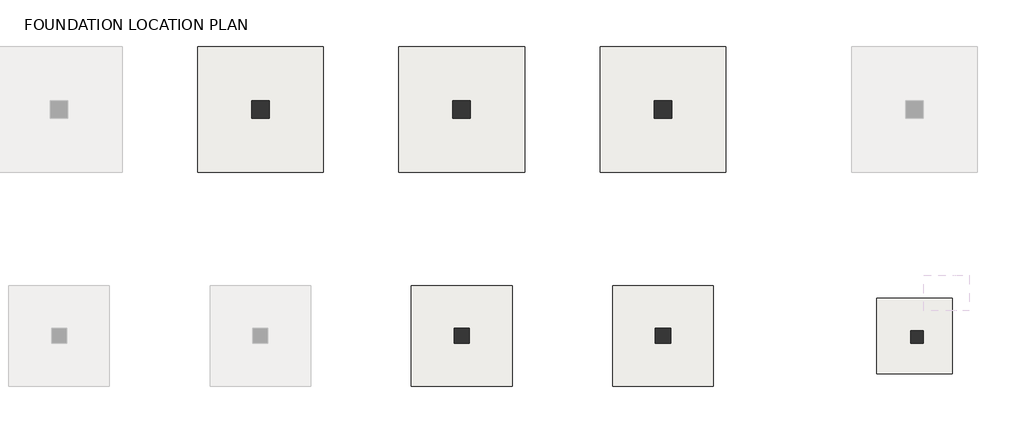
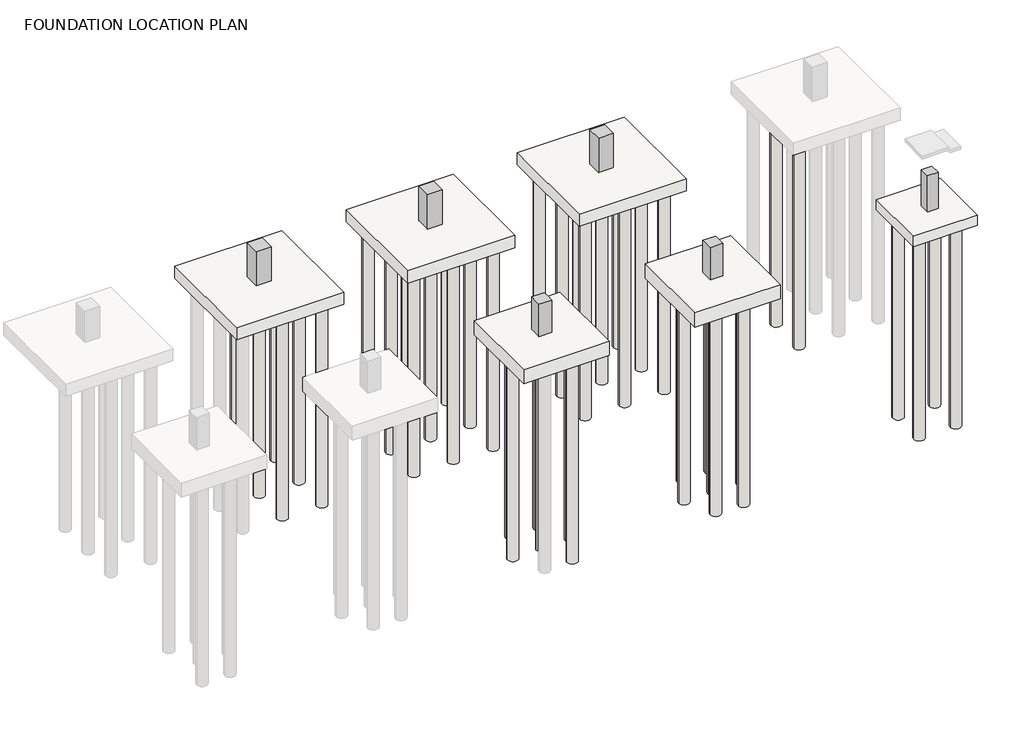
# One storey, part 2 of 3: 49 slabs, 6 columns.
"""IFC4 building model written with IfcOpenShell, lengths in millimetres."""

import ifcopenshell
import ifcopenshell.guid

model = None  # the IFC model being written
_history = None  # IfcOwnerHistory: only IFC2X3 demands one
_inside = {}  # id of a spatial element -> (the spatial element, [elements in it])
_under = {}  # id of a project, library or spatial element -> (it, [spatial elements below it])
_declared = {}  # id of a project -> (the project, [libraries it declares])
_typed = {}  # id of a type object -> (the type object, [elements of that type])
_made_of = {}  # id of a material, layer set ... -> (it, [elements and type objects made of it])


def new_model(schema):
    """Start an empty IFC model of exactly this schema.

    Asked for "IFC4X3", IfcOpenShell would pick the latest addendum, in which some entities
    have other attributes; the version numbers below select the first issue.
    IFC2X3 requires an IfcOwnerHistory on every rooted entity: one is made here for all.
    """
    global model, _history
    if schema == "IFC4X3":
        model = ifcopenshell.file(schema_version=(4, 3, 0, 0))
    else:
        model = ifcopenshell.file(schema=schema)
    _inside.clear()
    _under.clear()
    _declared.clear()
    _typed.clear()
    _made_of.clear()
    _history = None
    if model.schema == "IFC2X3":
        org = make("IfcOrganization", Name="unknown")
        user = make(
            "IfcPersonAndOrganization",
            ThePerson=make("IfcPerson", FamilyName="unknown"),
            TheOrganization=org,
        )
        app = make(
            "IfcApplication",
            ApplicationDeveloper=org,
            Version="unknown",
            ApplicationFullName="unknown",
            ApplicationIdentifier="unknown",
        )
        _history = make(
            "IfcOwnerHistory",
            OwningUser=user,
            OwningApplication=app,
            ChangeAction="ADDED",
            CreationDate=0,
        )
    return model


def make(cls, **values):
    """One entity of the class cls with the attributes given. An attribute that is None is left unset."""
    return model.create_entity(
        cls, **{name: value for name, value in values.items() if value is not None}
    )


def rooted(cls, **values):
    """An entity with a GlobalId (a new one), such as an element, a storey or a relation."""
    return make(cls, GlobalId=ifcopenshell.guid.new(), OwnerHistory=_history, **values)


def si_unit(unit_type, name, prefix=None):
    """IfcSIUnit, for example si_unit("LENGTHUNIT", "METRE", prefix="MILLI")."""
    return make("IfcSIUnit", UnitType=unit_type, Prefix=prefix, Name=name)


def assignment(units):
    """IfcUnitAssignment: the units of a project."""
    return None if units is None else make("IfcUnitAssignment", Units=units)


def point(xyz):
    """IfcCartesianPoint."""
    return None if xyz is None else make("IfcCartesianPoint", Coordinates=xyz)


def direction(xyz):
    """IfcDirection."""
    return None if xyz is None else make("IfcDirection", DirectionRatios=xyz)


def frame(location, z_axis=None, x_axis=None):
    """IfcAxis2Placement3D, a coordinate frame: its origin and axes. An axis left out is left unset."""
    return make(
        "IfcAxis2Placement3D",
        Location=point(location),
        Axis=direction(z_axis),
        RefDirection=direction(x_axis),
    )


def frame_2d(location, x_axis=None):
    """IfcAxis2Placement2D, a coordinate frame in the plane: its origin and x axis."""
    return make(
        "IfcAxis2Placement2D", Location=point(location), RefDirection=direction(x_axis)
    )


def origin():
    """The frame at (0, 0, 0) with its axes left unset."""
    return frame((0.0, 0.0, 0.0))


def place(relative_to, where):
    """IfcLocalPlacement: puts the frame where relative to a parent placement (None: the world)."""
    return make(
        "IfcLocalPlacement", PlacementRelTo=relative_to, RelativePlacement=where
    )


def context(
    kind, dimensions, precision=None, world=None, true_north=None, identifier=None
):
    """IfcGeometricRepresentationContext, for example the 3D "Model" context."""
    return make(
        "IfcGeometricRepresentationContext",
        ContextIdentifier=identifier,
        ContextType=kind,
        CoordinateSpaceDimension=dimensions,
        Precision=precision,
        WorldCoordinateSystem=world,
        TrueNorth=true_north,
    )


def project(units=None, contexts=None):
    """IfcProject with its units and contexts."""
    return rooted(
        "IfcProject",
        Name="project",
        RepresentationContexts=contexts,
        UnitsInContext=assignment(units),
    )


def spatial(cls, under=None, at=None, **own):
    """A site, building, storey or space (cls), placed at a placement, below another one or the project."""
    s = rooted(cls, ObjectPlacement=at, **own)
    if under is not None:
        _under.setdefault(under.id(), (under, []))[1].append(s)
    return s


def polyline(points):
    """IfcPolyline through the points."""
    return make("IfcPolyline", Points=[point(p) for p in points])


def circle_curve(where, radius):
    """IfcCircle in the frame where."""
    return make("IfcCircle", Position=where, Radius=radius)


def trimmed(basis, trim1, trim2, sense, master):
    """IfcTrimmedCurve: the piece of a basis curve between two trims."""
    return make(
        "IfcTrimmedCurve",
        BasisCurve=basis,
        Trim1=trim1,
        Trim2=trim2,
        SenseAgreement=sense,
        MasterRepresentation=master,
    )


def segment(curve, same_sense, transition):
    """IfcCompositeCurveSegment."""
    return make(
        "IfcCompositeCurveSegment",
        Transition=transition,
        SameSense=same_sense,
        ParentCurve=curve,
    )


def composite_curve(segments, self_intersect=None):
    """IfcCompositeCurve: segments joined end to end."""
    return make("IfcCompositeCurve", Segments=segments, SelfIntersect=self_intersect)


def outline(outer, holes=None, kind="AREA"):
    """IfcArbitraryClosedProfileDef: a profile drawn as a closed curve; with holes, ...WithVoids."""
    if holes is None:
        return make("IfcArbitraryClosedProfileDef", ProfileType=kind, OuterCurve=outer)
    return make(
        "IfcArbitraryProfileDefWithVoids",
        ProfileType=kind,
        OuterCurve=outer,
        InnerCurves=holes,
    )


def extrude(swept, where, along, depth):
    """IfcExtrudedAreaSolid: the profile swept, set in the frame where, extruded along a direction by depth."""
    return make(
        "IfcExtrudedAreaSolid",
        SweptArea=swept,
        Position=where,
        ExtrudedDirection=direction(along),
        Depth=depth,
    )


def faces_of(points, faces, orient=None, outer=None):
    """IfcFace entities. A face is a list of loops; a loop is a list of indices into points, from 0.

    orient and outer hold one flag for each loop. By default every Orientation is true, the
    first loop of a face is its IfcFaceOuterBound and the others are IfcFaceBound.
    """
    made = []
    for i, loops in enumerate(faces):
        bounds = []
        for j, loop in enumerate(loops):
            is_outer = j == 0 if outer is None else outer[i][j]
            bounds.append(
                make(
                    "IfcFaceOuterBound" if is_outer else "IfcFaceBound",
                    Bound=make("IfcPolyLoop", Polygon=[points[k] for k in loop]),
                    Orientation=True if orient is None else orient[i][j],
                )
            )
        made.append(make("IfcFace", Bounds=bounds))
    return made


def faceted_brep(points, faces, orient=None, outer=None, voids=None):
    """IfcFacetedBrep: a solid bounded by flat faces; with voids (closed shells), ...WithVoids."""
    shared = [point(p) for p in points]
    hull = make("IfcClosedShell", CfsFaces=faces_of(shared, faces, orient, outer))
    if voids is None:
        return make("IfcFacetedBrep", Outer=hull)
    return make(
        "IfcFacetedBrepWithVoids",
        Outer=hull,
        Voids=[
            make(cls, CfsFaces=faces_of(shared, fs, o, b)) for cls, fs, o, b in voids
        ],
    )


def shape(context_of_items, identifier, shape_type, items):
    """IfcShapeRepresentation: the items that make up one representation, for example the "Body"."""
    return make(
        "IfcShapeRepresentation",
        ContextOfItems=context_of_items,
        RepresentationIdentifier=identifier,
        RepresentationType=shape_type,
        Items=items,
    )


def made_of(thing, what):
    """Note that an element or type object is made of a material, layer set ...; save() writes the relation."""
    if what is not None:
        _made_of.setdefault(what.id(), (what, []))[1].append(thing)
    return thing


def element(
    cls,
    number,
    at=None,
    inside=None,
    cuts=None,
    type_object=None,
    material=None,
    context=None,
    identifier="Body",
    shape_type=None,
    held_by="IfcProductDefinitionShape",
    body=None,
    shapes=None,
    **own,
):
    """One element of the class cls, such as IfcWall. Its Tag is "e" and its number.

    at: its placement. inside: the storey or other place that contains it. cuts: it is an
    opening in that element (IfcRelVoidsElement). A single representation is given by context,
    identifier, shape_type and body (its items); several are given by shapes. held_by: the class
    of the entity that holds the representations. save() writes the other relations.
    """
    e = rooted(cls, Tag="e%d" % number, ObjectPlacement=at, **own)
    if body is not None:
        shapes = [shape(context, identifier, shape_type, body)]
    if shapes is not None:
        e.Representation = make(held_by, Representations=shapes)
    if inside is not None:
        _inside.setdefault(inside.id(), (inside, []))[1].append(e)
    if cuts is not None:
        rooted(
            "IfcRelVoidsElement", RelatingBuildingElement=cuts, RelatedOpeningElement=e
        )
    if type_object is not None:
        _typed.setdefault(type_object.id(), (type_object, []))[1].append(e)
    return made_of(e, material)


def aggregate(whole, parts):
    """IfcRelAggregates: a whole, such as a stair, and the parts it consists of."""
    return rooted("IfcRelAggregates", RelatingObject=whole, RelatedObjects=parts)


def save(model, path):
    """Write the relations noted so far, then the file.

    IfcRelAggregates (storeys below a building ...), IfcRelContainedInSpatialStructure (elements
    in a storey), IfcRelDefinesByType, IfcRelAssociatesMaterial and IfcRelDeclares: one each for
    every whole, place, type object, material and project.
    """
    for whole, parts in _under.values():
        aggregate(whole, parts)
    for where, things in _inside.values():
        rooted(
            "IfcRelContainedInSpatialStructure",
            RelatedElements=things,
            RelatingStructure=where,
        )
    for kind, things in _typed.values():
        rooted("IfcRelDefinesByType", RelatedObjects=things, RelatingType=kind)
    for what, things in _made_of.values():
        rooted("IfcRelAssociatesMaterial", RelatedObjects=things, RelatingMaterial=what)
    for by, libraries in _declared.values():
        rooted("IfcRelDeclares", RelatingContext=by, RelatedDefinitions=libraries)
    model.write(path)


model = new_model("IFC4")

# Units and contexts
model_context = context("Model", 3, world=origin())
ifc_project = project(units=[si_unit("LENGTHUNIT", "METRE", prefix="MILLI")], contexts=[model_context])

# Site, building, storey
site = spatial("IfcSite", under=ifc_project)
building = spatial("IfcBuilding", under=site)
storey = spatial("IfcBuildingStorey", under=building, Name="FOUNDATION LOCATION PLAN", Elevation=-1699.994759)

# Columns
placement = place(None, origin())
element("IfcColumn", 1, ObjectType="Concrete-Rectangular-Column_R1 : CLS111_RC COLUMN_UG_C1", at=placement, inside=storey, context=model_context, shape_type="Brep", body=[
    faceted_brep([(41850.0, 21199.5208589, -1199.994759), (42350.0, 21199.5208589, -1199.994759), (42350.0, 20699.5208589, -1199.994759), (41850.0, 20699.5208589, -1199.994759), (41850.0, 21199.5208589, 450.005241), (41850.0, 21199.5208589, 600.005241), (42000.0, 21199.5208589, 600.005241), (42350.0, 21199.5208589, 600.005241), (41850.0, 20699.5208589, 600.005241), (41850.0, 20999.5208589, 600.005241), (42350.0, 20699.5208589, 600.005241)], [[[0, 1, 2, 3]], [[1, 0, 4, 5, 6, 7]], [[0, 3, 8, 9, 5, 4]], [[3, 2, 10, 8]], [[2, 1, 7, 10]], [[8, 10, 7, 6, 5, 9]]]),
])
element("IfcColumn", 2, ObjectType="Concrete-Rectangular-Column_R1 : CLS111_RC COLUMN_UG_C3", at=placement, inside=storey, context=model_context, shape_type="Brep", body=[
    faceted_brep([(15650.0, 30349.5208589, -1099.994759), (16350.0, 30349.5208589, -1099.994759), (16350.0, 29649.5208589, -1099.994759), (15650.0, 29649.5208589, -1099.994759), (15650.0, 30349.5208589, 450.005241), (15650.0, 30349.5208589, 600.005241), (16350.0, 30349.5208589, 600.005241), (16350.0, 30349.5208589, 450.005241), (16350.0, 29649.5208589, 600.005241), (16350.0, 29649.5208589, 450.005241), (15650.0, 29649.5208589, 600.005241), (15650.0, 29649.5208589, 450.005241)], [[[0, 1, 2, 3]], [[1, 0, 4, 5, 6, 7]], [[2, 1, 7, 6, 8, 9]], [[3, 2, 9, 8, 10, 11]], [[0, 3, 11, 10, 5, 4]], [[6, 5, 10, 8]]]),
])
element("IfcColumn", 3, ObjectType="Concrete-Rectangular-Column_R1 : CLS111_RC COLUMN_UG_C3", at=placement, inside=storey, context=model_context, shape_type="Brep", body=[
    faceted_brep([(23650.0, 30349.5208589, -1099.994759), (24350.0, 30349.5208589, -1099.994759), (24350.0, 29649.5208589, -1099.994759), (23650.0, 29649.5208589, -1099.994759), (23650.0, 30349.5208589, 450.005241), (23650.0, 30349.5208589, 600.005241), (24350.0, 30349.5208589, 600.005241), (24350.0, 30349.5208589, 450.005241), (24350.0, 29649.5208589, 600.005241), (24350.0, 29649.5208589, 450.005241), (23650.0, 29649.5208589, 600.005241), (23650.0, 29649.5208589, 450.005241)], [[[0, 1, 2, 3]], [[1, 0, 4, 5, 6, 7]], [[2, 1, 7, 6, 8, 9]], [[3, 2, 9, 8, 10, 11]], [[0, 3, 11, 10, 5, 4]], [[6, 5, 10, 8]]]),
])
element("IfcColumn", 4, ObjectType="Concrete-Rectangular-Column_R1 : CLS111_RC COLUMN_UG_C3", at=placement, inside=storey, context=model_context, shape_type="Brep", body=[
    faceted_brep([(31650.0, 30349.5208589, -1099.994759), (32350.0, 30349.5208589, -1099.994759), (32350.0, 29649.5208589, -1099.994759), (31650.0, 29649.5208589, -1099.994759), (31650.0, 30349.5208589, 450.005241), (31650.0, 30349.5208589, 600.005241), (32350.0, 30349.5208589, 600.005241), (32350.0, 30349.5208589, 450.005241), (32350.0, 29649.5208589, 600.005241), (32350.0, 29649.5208589, 450.005241), (31650.0, 29649.5208589, 600.005241), (31650.0, 29649.5208589, 450.005241)], [[[0, 1, 2, 3]], [[1, 0, 4, 5, 6, 7]], [[2, 1, 7, 6, 8, 9]], [[3, 2, 9, 8, 10, 11]], [[0, 3, 11, 10, 5, 4]], [[6, 5, 10, 8]]]),
])
element("IfcColumn", 5, ObjectType="Concrete-Rectangular-Column_R1 : CLS111_RC COLUMN_UG_C2", at=placement, inside=storey, context=model_context, shape_type="Brep", body=[
    faceted_brep([(23700.0, 21299.5208589, -999.994759), (24300.0, 21299.5208589, -999.994759), (24300.0, 20699.5208589, -999.994759), (23700.0, 20699.5208589, -999.994759), (23700.0, 21299.5208589, 450.005241), (23700.0, 21299.5208589, 600.005241), (24300.0, 21299.5208589, 600.005241), (24300.0, 21299.5208589, 450.005241), (24300.0, 20999.5208589, 600.005241), (24300.0, 20699.5208589, 600.005241), (23700.0, 20699.5208589, 600.005241), (23700.0, 20999.5208589, 600.005241)], [[[0, 1, 2, 3]], [[1, 0, 4, 5, 6, 7]], [[2, 1, 7, 6, 8, 9]], [[3, 2, 9, 10]], [[0, 3, 10, 11, 5, 4]], [[6, 5, 11, 10, 9, 8]]]),
])
element("IfcColumn", 6, ObjectType="Concrete-Rectangular-Column_R1 : CLS111_RC COLUMN_UG_C2", at=placement, inside=storey, context=model_context, shape_type="Brep", body=[
    faceted_brep([(31700.0, 21299.5208589, -999.994759), (32300.0, 21299.5208589, -999.994759), (32300.0, 20699.5208589, -999.994759), (31700.0, 20699.5208589, -999.994759), (31700.0, 21299.5208589, 450.005241), (31700.0, 21299.5208589, 600.005241), (32300.0, 21299.5208589, 600.005241), (32300.0, 21299.5208589, 450.005241), (32300.0, 20999.5208589, 600.005241), (32300.0, 20699.5208589, 600.005241), (31700.0, 20699.5208589, 600.005241), (31700.0, 20999.5208589, 600.005241)], [[[0, 1, 2, 3]], [[1, 0, 4, 5, 6, 7]], [[2, 1, 7, 6, 8, 9]], [[3, 2, 9, 10]], [[0, 3, 10, 11, 5, 4]], [[6, 5, 11, 10, 9, 8]]]),
])

# Slabs
element("IfcSlab", 7, ObjectType="Footing-Rectangular_R1 : FTS301_Footing-Rectangular_3000x3000x500_F1", at=placement, inside=storey, context=model_context, shape_type="SweptSolid", body=[
    extrude(outline(polyline([(43500.0, 22499.5208589), (43500.0, 19499.5208589), (40500.0, 19499.5208589), (40500.0, 22499.5208589), (43500.0, 22499.5208589)])), frame((0.0, 0.0, -1699.994759), z_axis=(0.0, 0.0, 1.0), x_axis=(1.0, 0.0, 0.0)), (0.0, 0.0, 1.0), 500.0),
])
element("IfcSlab", 8, ObjectType="Footing-Rectangular_R1 : FTS301_Footing-Rectangular_4000x4000x700_F2", at=placement, inside=storey, context=model_context, shape_type="SweptSolid", body=[
    extrude(outline(polyline([(26000.0, 22999.5208589), (26000.0, 18999.5208589), (22000.0, 18999.5208589), (22000.0, 22999.5208589), (26000.0, 22999.5208589)])), frame((0.0, 0.0, -1699.994759), z_axis=(0.0, 0.0, 1.0), x_axis=(1.0, 0.0, 0.0)), (0.0, 0.0, 1.0), 700.0),
])
element("IfcSlab", 9, ObjectType="Footing-Rectangular_R1 : FTS301_Footing-Rectangular_4000x4000x700_F2", at=placement, inside=storey, context=model_context, shape_type="SweptSolid", body=[
    extrude(outline(polyline([(34000.0, 22999.5208589), (34000.0, 18999.5208589), (30000.0, 18999.5208589), (30000.0, 22999.5208589), (34000.0, 22999.5208589)])), frame((0.0, 0.0, -1699.994759), z_axis=(0.0, 0.0, 1.0), x_axis=(1.0, 0.0, 0.0)), (0.0, 0.0, 1.0), 700.0),
])
element("IfcSlab", 10, ObjectType="Footing-Rectangular_R1 : FTS301_Footing-Rectangular_5000x5000x600_F3", at=placement, inside=storey, context=model_context, shape_type="SweptSolid", body=[
    extrude(outline(polyline([(18500.0, 32499.5208589), (18500.0, 27499.5208589), (13500.0, 27499.5208589), (13500.0, 32499.5208589), (18500.0, 32499.5208589)])), frame((0.0, 0.0, -1699.994759), z_axis=(0.0, 0.0, 1.0), x_axis=(1.0, 0.0, 0.0)), (0.0, 0.0, 1.0), 600.0),
])
element("IfcSlab", 11, ObjectType="Footing-Rectangular_R1 : FTS301_Footing-Rectangular_5000x5000x600_F3", at=placement, inside=storey, context=model_context, shape_type="SweptSolid", body=[
    extrude(outline(polyline([(26500.0, 32499.5208589), (26500.0, 27499.5208589), (21500.0, 27499.5208589), (21500.0, 32499.5208589), (26500.0, 32499.5208589)])), frame((0.0, 0.0, -1699.994759), z_axis=(0.0, 0.0, 1.0), x_axis=(1.0, 0.0, 0.0)), (0.0, 0.0, 1.0), 600.0),
])
element("IfcSlab", 12, ObjectType="Footing-Rectangular_R1 : FTS301_Footing-Rectangular_5000x5000x600_F3", at=placement, inside=storey, context=model_context, shape_type="SweptSolid", body=[
    extrude(outline(polyline([(34500.0, 32499.5208589), (34500.0, 27499.5208589), (29500.0, 27499.5208589), (29500.0, 32499.5208589), (34500.0, 32499.5208589)])), frame((0.0, 0.0, -1699.994759), z_axis=(0.0, 0.0, 1.0), x_axis=(1.0, 0.0, 0.0)), (0.0, 0.0, 1.0), 600.0),
])
element("IfcSlab", 13, ObjectType="HEC_PILE : FTPS102_D500", at=placement, inside=storey, context=model_context, shape_type="SweptSolid", body=[
    extrude(outline(composite_curve([segment(trimmed(circle_curve(frame_2d((41150.0, 21849.5208589)), 250.0), [point((41400.0, 21849.5208589))], [point((40900.0, 21849.5208589))], False, "CARTESIAN"), True, "CONTINUOUS"), segment(trimmed(circle_curve(frame_2d((41150.0, 21849.5208589)), 250.0), [point((40900.0, 21849.5208589))], [point((41400.0, 21849.5208589))], False, "CARTESIAN"), True, "CONTINUOUS")], self_intersect=False)), frame((0.0, 0.0, -11749.994759), z_axis=(0.0, 0.0, 1.0), x_axis=(1.0, 0.0, 0.0)), (0.0, 0.0, 1.0), 10150.0),
])
element("IfcSlab", 14, ObjectType="HEC_PILE : FTPS102_D500", at=placement, inside=storey, context=model_context, shape_type="SweptSolid", body=[
    extrude(outline(composite_curve([segment(trimmed(circle_curve(frame_2d((42850.0, 21849.5208589)), 250.0), [point((42600.0, 21849.5208589))], [point((43100.0, 21849.5208589))], False, "CARTESIAN"), True, "CONTINUOUS"), segment(trimmed(circle_curve(frame_2d((42850.0, 21849.5208589)), 250.0), [point((43100.0, 21849.5208589))], [point((42600.0, 21849.5208589))], False, "CARTESIAN"), True, "CONTINUOUS")], self_intersect=False)), frame((0.0, 0.0, -11749.994759), z_axis=(0.0, 0.0, 1.0), x_axis=(1.0, 0.0, 0.0)), (0.0, 0.0, 1.0), 10150.0),
])
element("IfcSlab", 15, ObjectType="HEC_PILE : FTPS102_D500", at=placement, inside=storey, context=model_context, shape_type="SweptSolid", body=[
    extrude(outline(composite_curve([segment(trimmed(circle_curve(frame_2d((41150.0, 20149.5208589)), 250.0), [point((41400.0, 20149.5208589))], [point((40900.0, 20149.5208589))], False, "CARTESIAN"), True, "CONTINUOUS"), segment(trimmed(circle_curve(frame_2d((41150.0, 20149.5208589)), 250.0), [point((40900.0, 20149.5208589))], [point((41400.0, 20149.5208589))], False, "CARTESIAN"), True, "CONTINUOUS")], self_intersect=False)), frame((0.0, 0.0, -11749.994759), z_axis=(0.0, 0.0, 1.0), x_axis=(1.0, 0.0, 0.0)), (0.0, 0.0, 1.0), 10150.0),
])
element("IfcSlab", 16, ObjectType="HEC_PILE : FTPS102_D500", at=placement, inside=storey, context=model_context, shape_type="SweptSolid", body=[
    extrude(outline(composite_curve([segment(trimmed(circle_curve(frame_2d((42850.0, 20149.5208589)), 250.0), [point((42600.0, 20149.5208589))], [point((43100.0, 20149.5208589))], False, "CARTESIAN"), True, "CONTINUOUS"), segment(trimmed(circle_curve(frame_2d((42850.0, 20149.5208589)), 250.0), [point((43100.0, 20149.5208589))], [point((42600.0, 20149.5208589))], False, "CARTESIAN"), True, "CONTINUOUS")], self_intersect=False)), frame((0.0, 0.0, -11749.994759), z_axis=(0.0, 0.0, 1.0), x_axis=(1.0, 0.0, 0.0)), (0.0, 0.0, 1.0), 10150.0),
])
element("IfcSlab", 17, ObjectType="HEC_PILE : FTPS102_D500", at=placement, inside=storey, context=model_context, shape_type="SweptSolid", body=[
    extrude(outline(composite_curve([segment(trimmed(circle_curve(frame_2d((24650.0, 19649.5208589)), 250.0), [point((24400.0, 19649.5208589))], [point((24900.0, 19649.5208589))], False, "CARTESIAN"), True, "CONTINUOUS"), segment(trimmed(circle_curve(frame_2d((24650.0, 19649.5208589)), 250.0), [point((24900.0, 19649.5208589))], [point((24400.0, 19649.5208589))], False, "CARTESIAN"), True, "CONTINUOUS")], self_intersect=False)), frame((0.0, 0.0, -11749.994759), z_axis=(0.0, 0.0, 1.0), x_axis=(1.0, 0.0, 0.0)), (0.0, 0.0, 1.0), 10150.0),
])
element("IfcSlab", 18, ObjectType="HEC_PILE : FTPS102_D500", at=placement, inside=storey, context=model_context, shape_type="SweptSolid", body=[
    extrude(outline(composite_curve([segment(trimmed(circle_curve(frame_2d((22650.0, 20999.5208589)), 250.0), [point((22900.0, 20999.5208589))], [point((22400.0, 20999.5208589))], False, "CARTESIAN"), True, "CONTINUOUS"), segment(trimmed(circle_curve(frame_2d((22650.0, 20999.5208589)), 250.0), [point((22400.0, 20999.5208589))], [point((22900.0, 20999.5208589))], False, "CARTESIAN"), True, "CONTINUOUS")], self_intersect=False)), frame((0.0, 0.0, -11749.994759), z_axis=(0.0, 0.0, 1.0), x_axis=(1.0, 0.0, 0.0)), (0.0, 0.0, 1.0), 10150.0),
])
element("IfcSlab", 19, ObjectType="HEC_PILE : FTPS102_D500", at=placement, inside=storey, context=model_context, shape_type="SweptSolid", body=[
    extrude(outline(composite_curve([segment(trimmed(circle_curve(frame_2d((24000.0, 20999.5208589)), 250.0), [point((24250.0, 20999.5208589))], [point((23750.0, 20999.5208589))], False, "CARTESIAN"), True, "CONTINUOUS"), segment(trimmed(circle_curve(frame_2d((24000.0, 20999.5208589)), 250.0), [point((23750.0, 20999.5208589))], [point((24250.0, 20999.5208589))], False, "CARTESIAN"), True, "CONTINUOUS")], self_intersect=False)), frame((0.0, 0.0, -11749.994759), z_axis=(0.0, 0.0, 1.0), x_axis=(1.0, 0.0, 0.0)), (0.0, 0.0, 1.0), 10150.0),
])
element("IfcSlab", 20, ObjectType="HEC_PILE : FTPS102_D500", at=placement, inside=storey, context=model_context, shape_type="SweptSolid", body=[
    extrude(outline(composite_curve([segment(trimmed(circle_curve(frame_2d((25350.0, 20999.5208589)), 250.0), [point((25100.0, 20999.5208589))], [point((25600.0, 20999.5208589))], False, "CARTESIAN"), True, "CONTINUOUS"), segment(trimmed(circle_curve(frame_2d((25350.0, 20999.5208589)), 250.0), [point((25600.0, 20999.5208589))], [point((25100.0, 20999.5208589))], False, "CARTESIAN"), True, "CONTINUOUS")], self_intersect=False)), frame((0.0, 0.0, -11749.994759), z_axis=(0.0, 0.0, 1.0), x_axis=(1.0, 0.0, 0.0)), (0.0, 0.0, 1.0), 10150.0),
])
element("IfcSlab", 21, ObjectType="HEC_PILE : FTPS102_D500", at=placement, inside=storey, context=model_context, shape_type="SweptSolid", body=[
    extrude(outline(composite_curve([segment(trimmed(circle_curve(frame_2d((23350.0, 22349.5208589)), 250.0), [point((23600.0, 22349.5208589))], [point((23100.0, 22349.5208589))], False, "CARTESIAN"), True, "CONTINUOUS"), segment(trimmed(circle_curve(frame_2d((23350.0, 22349.5208589)), 250.0), [point((23100.0, 22349.5208589))], [point((23600.0, 22349.5208589))], False, "CARTESIAN"), True, "CONTINUOUS")], self_intersect=False)), frame((0.0, 0.0, -11749.994759), z_axis=(0.0, 0.0, 1.0), x_axis=(1.0, 0.0, 0.0)), (0.0, 0.0, 1.0), 10150.0),
])
element("IfcSlab", 22, ObjectType="HEC_PILE : FTPS102_D500", at=placement, inside=storey, context=model_context, shape_type="SweptSolid", body=[
    extrude(outline(composite_curve([segment(trimmed(circle_curve(frame_2d((24650.0, 22349.5208589)), 250.0), [point((24400.0, 22349.5208589))], [point((24900.0, 22349.5208589))], False, "CARTESIAN"), True, "CONTINUOUS"), segment(trimmed(circle_curve(frame_2d((24650.0, 22349.5208589)), 250.0), [point((24900.0, 22349.5208589))], [point((24400.0, 22349.5208589))], False, "CARTESIAN"), True, "CONTINUOUS")], self_intersect=False)), frame((0.0, 0.0, -11749.994759), z_axis=(0.0, 0.0, 1.0), x_axis=(1.0, 0.0, 0.0)), (0.0, 0.0, 1.0), 10150.0),
])
element("IfcSlab", 23, ObjectType="HEC_PILE : FTPS102_D500", at=placement, inside=storey, context=model_context, shape_type="SweptSolid", body=[
    extrude(outline(composite_curve([segment(trimmed(circle_curve(frame_2d((31350.0, 19649.5208589)), 250.0), [point((31600.0, 19649.5208589))], [point((31100.0, 19649.5208589))], False, "CARTESIAN"), True, "CONTINUOUS"), segment(trimmed(circle_curve(frame_2d((31350.0, 19649.5208589)), 250.0), [point((31100.0, 19649.5208589))], [point((31600.0, 19649.5208589))], False, "CARTESIAN"), True, "CONTINUOUS")], self_intersect=False)), frame((0.0, 0.0, -11749.994759), z_axis=(0.0, 0.0, 1.0), x_axis=(1.0, 0.0, 0.0)), (0.0, 0.0, 1.0), 10150.0),
])
element("IfcSlab", 24, ObjectType="HEC_PILE : FTPS102_D500", at=placement, inside=storey, context=model_context, shape_type="SweptSolid", body=[
    extrude(outline(composite_curve([segment(trimmed(circle_curve(frame_2d((32650.0, 19649.5208589)), 250.0), [point((32400.0, 19649.5208589))], [point((32900.0, 19649.5208589))], False, "CARTESIAN"), True, "CONTINUOUS"), segment(trimmed(circle_curve(frame_2d((32650.0, 19649.5208589)), 250.0), [point((32900.0, 19649.5208589))], [point((32400.0, 19649.5208589))], False, "CARTESIAN"), True, "CONTINUOUS")], self_intersect=False)), frame((0.0, 0.0, -11749.994759), z_axis=(0.0, 0.0, 1.0), x_axis=(1.0, 0.0, 0.0)), (0.0, 0.0, 1.0), 10150.0),
])
element("IfcSlab", 25, ObjectType="HEC_PILE : FTPS102_D500", at=placement, inside=storey, context=model_context, shape_type="SweptSolid", body=[
    extrude(outline(composite_curve([segment(trimmed(circle_curve(frame_2d((30650.0, 20999.5208589)), 250.0), [point((30900.0, 20999.5208589))], [point((30400.0, 20999.5208589))], False, "CARTESIAN"), True, "CONTINUOUS"), segment(trimmed(circle_curve(frame_2d((30650.0, 20999.5208589)), 250.0), [point((30400.0, 20999.5208589))], [point((30900.0, 20999.5208589))], False, "CARTESIAN"), True, "CONTINUOUS")], self_intersect=False)), frame((0.0, 0.0, -11749.994759), z_axis=(0.0, 0.0, 1.0), x_axis=(1.0, 0.0, 0.0)), (0.0, 0.0, 1.0), 10150.0),
])
element("IfcSlab", 26, ObjectType="HEC_PILE : FTPS102_D500", at=placement, inside=storey, context=model_context, shape_type="SweptSolid", body=[
    extrude(outline(composite_curve([segment(trimmed(circle_curve(frame_2d((32000.0, 20999.5208589)), 250.0), [point((32250.0, 20999.5208589))], [point((31750.0, 20999.5208589))], False, "CARTESIAN"), True, "CONTINUOUS"), segment(trimmed(circle_curve(frame_2d((32000.0, 20999.5208589)), 250.0), [point((31750.0, 20999.5208589))], [point((32250.0, 20999.5208589))], False, "CARTESIAN"), True, "CONTINUOUS")], self_intersect=False)), frame((0.0, 0.0, -11749.994759), z_axis=(0.0, 0.0, 1.0), x_axis=(1.0, 0.0, 0.0)), (0.0, 0.0, 1.0), 10150.0),
])
element("IfcSlab", 27, ObjectType="HEC_PILE : FTPS102_D500", at=placement, inside=storey, context=model_context, shape_type="SweptSolid", body=[
    extrude(outline(composite_curve([segment(trimmed(circle_curve(frame_2d((33350.0, 20999.5208589)), 250.0), [point((33100.0, 20999.5208589))], [point((33600.0, 20999.5208589))], False, "CARTESIAN"), True, "CONTINUOUS"), segment(trimmed(circle_curve(frame_2d((33350.0, 20999.5208589)), 250.0), [point((33600.0, 20999.5208589))], [point((33100.0, 20999.5208589))], False, "CARTESIAN"), True, "CONTINUOUS")], self_intersect=False)), frame((0.0, 0.0, -11749.994759), z_axis=(0.0, 0.0, 1.0), x_axis=(1.0, 0.0, 0.0)), (0.0, 0.0, 1.0), 10150.0),
])
element("IfcSlab", 28, ObjectType="HEC_PILE : FTPS102_D500", at=placement, inside=storey, context=model_context, shape_type="SweptSolid", body=[
    extrude(outline(composite_curve([segment(trimmed(circle_curve(frame_2d((31350.0, 22349.5208589)), 250.0), [point((31600.0, 22349.5208589))], [point((31100.0, 22349.5208589))], False, "CARTESIAN"), True, "CONTINUOUS"), segment(trimmed(circle_curve(frame_2d((31350.0, 22349.5208589)), 250.0), [point((31100.0, 22349.5208589))], [point((31600.0, 22349.5208589))], False, "CARTESIAN"), True, "CONTINUOUS")], self_intersect=False)), frame((0.0, 0.0, -11749.994759), z_axis=(0.0, 0.0, 1.0), x_axis=(1.0, 0.0, 0.0)), (0.0, 0.0, 1.0), 10150.0),
])
element("IfcSlab", 29, ObjectType="HEC_PILE : FTPS102_D500", at=placement, inside=storey, context=model_context, shape_type="SweptSolid", body=[
    extrude(outline(composite_curve([segment(trimmed(circle_curve(frame_2d((32650.0, 22349.5208589)), 250.0), [point((32400.0, 22349.5208589))], [point((32900.0, 22349.5208589))], False, "CARTESIAN"), True, "CONTINUOUS"), segment(trimmed(circle_curve(frame_2d((32650.0, 22349.5208589)), 250.0), [point((32900.0, 22349.5208589))], [point((32400.0, 22349.5208589))], False, "CARTESIAN"), True, "CONTINUOUS")], self_intersect=False)), frame((0.0, 0.0, -11749.994759), z_axis=(0.0, 0.0, 1.0), x_axis=(1.0, 0.0, 0.0)), (0.0, 0.0, 1.0), 10150.0),
])
element("IfcSlab", 30, ObjectType="HEC_PILE : FTPS102_D500", at=placement, inside=storey, context=model_context, shape_type="SweptSolid", body=[
    extrude(outline(composite_curve([segment(trimmed(circle_curve(frame_2d((17850.0, 29999.5208589)), 250.0), [point((17600.0, 29999.5208589))], [point((18100.0, 29999.5208589))], False, "CARTESIAN"), True, "CONTINUOUS"), segment(trimmed(circle_curve(frame_2d((17850.0, 29999.5208589)), 250.0), [point((18100.0, 29999.5208589))], [point((17600.0, 29999.5208589))], False, "CARTESIAN"), True, "CONTINUOUS")], self_intersect=False)), frame((0.0, 0.0, -11749.994759), z_axis=(0.0, 0.0, 1.0), x_axis=(1.0, 0.0, 0.0)), (0.0, 0.0, 1.0), 10150.0),
])
element("IfcSlab", 31, ObjectType="HEC_PILE : FTPS102_D500", at=placement, inside=storey, context=model_context, shape_type="SweptSolid", body=[
    extrude(outline(composite_curve([segment(trimmed(circle_curve(frame_2d((16000.0, 29999.5208589)), 250.0), [point((15750.0, 29999.5208589))], [point((16250.0, 29999.5208589))], False, "CARTESIAN"), True, "CONTINUOUS"), segment(trimmed(circle_curve(frame_2d((16000.0, 29999.5208589)), 250.0), [point((16250.0, 29999.5208589))], [point((15750.0, 29999.5208589))], False, "CARTESIAN"), True, "CONTINUOUS")], self_intersect=False)), frame((0.0, 0.0, -11749.994759), z_axis=(0.0, 0.0, 1.0), x_axis=(1.0, 0.0, 0.0)), (0.0, 0.0, 1.0), 10150.0),
])
element("IfcSlab", 32, ObjectType="HEC_PILE : FTPS102_D500", at=placement, inside=storey, context=model_context, shape_type="SweptSolid", body=[
    extrude(outline(composite_curve([segment(trimmed(circle_curve(frame_2d((17850.0, 31849.5208589)), 250.0), [point((17600.0, 31849.5208589))], [point((18100.0, 31849.5208589))], False, "CARTESIAN"), True, "CONTINUOUS"), segment(trimmed(circle_curve(frame_2d((17850.0, 31849.5208589)), 250.0), [point((18100.0, 31849.5208589))], [point((17600.0, 31849.5208589))], False, "CARTESIAN"), True, "CONTINUOUS")], self_intersect=False)), frame((0.0, 0.0, -11749.994759), z_axis=(0.0, 0.0, 1.0), x_axis=(1.0, 0.0, 0.0)), (0.0, 0.0, 1.0), 10150.0),
])
element("IfcSlab", 33, ObjectType="HEC_PILE : FTPS102_D500", at=placement, inside=storey, context=model_context, shape_type="SweptSolid", body=[
    extrude(outline(composite_curve([segment(trimmed(circle_curve(frame_2d((16000.0, 31849.5208589)), 250.0), [point((15750.0, 31849.5208589))], [point((16250.0, 31849.5208589))], False, "CARTESIAN"), True, "CONTINUOUS"), segment(trimmed(circle_curve(frame_2d((16000.0, 31849.5208589)), 250.0), [point((16250.0, 31849.5208589))], [point((15750.0, 31849.5208589))], False, "CARTESIAN"), True, "CONTINUOUS")], self_intersect=False)), frame((0.0, 0.0, -11749.994759), z_axis=(0.0, 0.0, 1.0), x_axis=(1.0, 0.0, 0.0)), (0.0, 0.0, 1.0), 10150.0),
])
element("IfcSlab", 34, ObjectType="HEC_PILE : FTPS102_D500", at=placement, inside=storey, context=model_context, shape_type="SweptSolid", body=[
    extrude(outline(composite_curve([segment(trimmed(circle_curve(frame_2d((17850.0, 28149.5208589)), 250.0), [point((17600.0, 28149.5208589))], [point((18100.0, 28149.5208589))], False, "CARTESIAN"), True, "CONTINUOUS"), segment(trimmed(circle_curve(frame_2d((17850.0, 28149.5208589)), 250.0), [point((18100.0, 28149.5208589))], [point((17600.0, 28149.5208589))], False, "CARTESIAN"), True, "CONTINUOUS")], self_intersect=False)), frame((0.0, 0.0, -11749.994759), z_axis=(0.0, 0.0, 1.0), x_axis=(1.0, 0.0, 0.0)), (0.0, 0.0, 1.0), 10150.0),
])
element("IfcSlab", 35, ObjectType="HEC_PILE : FTPS102_D500", at=placement, inside=storey, context=model_context, shape_type="SweptSolid", body=[
    extrude(outline(composite_curve([segment(trimmed(circle_curve(frame_2d((16000.0, 28149.5208589)), 250.0), [point((15750.0, 28149.5208589))], [point((16250.0, 28149.5208589))], False, "CARTESIAN"), True, "CONTINUOUS"), segment(trimmed(circle_curve(frame_2d((16000.0, 28149.5208589)), 250.0), [point((16250.0, 28149.5208589))], [point((15750.0, 28149.5208589))], False, "CARTESIAN"), True, "CONTINUOUS")], self_intersect=False)), frame((0.0, 0.0, -11749.994759), z_axis=(0.0, 0.0, 1.0), x_axis=(1.0, 0.0, 0.0)), (0.0, 0.0, 1.0), 10150.0),
])
element("IfcSlab", 36, ObjectType="HEC_PILE : FTPS102_D500", at=placement, inside=storey, context=model_context, shape_type="SweptSolid", body=[
    extrude(outline(composite_curve([segment(trimmed(circle_curve(frame_2d((22150.0, 29999.5208589)), 250.0), [point((22400.0, 29999.5208589))], [point((21900.0, 29999.5208589))], False, "CARTESIAN"), True, "CONTINUOUS"), segment(trimmed(circle_curve(frame_2d((22150.0, 29999.5208589)), 250.0), [point((21900.0, 29999.5208589))], [point((22400.0, 29999.5208589))], False, "CARTESIAN"), True, "CONTINUOUS")], self_intersect=False)), frame((0.0, 0.0, -11749.994759), z_axis=(0.0, 0.0, 1.0), x_axis=(1.0, 0.0, 0.0)), (0.0, 0.0, 1.0), 10150.0),
])
element("IfcSlab", 37, ObjectType="HEC_PILE : FTPS102_D500", at=placement, inside=storey, context=model_context, shape_type="SweptSolid", body=[
    extrude(outline(composite_curve([segment(trimmed(circle_curve(frame_2d((25850.0, 29999.5208589)), 250.0), [point((25600.0, 29999.5208589))], [point((26100.0, 29999.5208589))], False, "CARTESIAN"), True, "CONTINUOUS"), segment(trimmed(circle_curve(frame_2d((25850.0, 29999.5208589)), 250.0), [point((26100.0, 29999.5208589))], [point((25600.0, 29999.5208589))], False, "CARTESIAN"), True, "CONTINUOUS")], self_intersect=False)), frame((0.0, 0.0, -11749.994759), z_axis=(0.0, 0.0, 1.0), x_axis=(1.0, 0.0, 0.0)), (0.0, 0.0, 1.0), 10150.0),
])
element("IfcSlab", 38, ObjectType="HEC_PILE : FTPS102_D500", at=placement, inside=storey, context=model_context, shape_type="SweptSolid", body=[
    extrude(outline(composite_curve([segment(trimmed(circle_curve(frame_2d((24000.0, 29999.5208589)), 250.0), [point((23750.0, 29999.5208589))], [point((24250.0, 29999.5208589))], False, "CARTESIAN"), True, "CONTINUOUS"), segment(trimmed(circle_curve(frame_2d((24000.0, 29999.5208589)), 250.0), [point((24250.0, 29999.5208589))], [point((23750.0, 29999.5208589))], False, "CARTESIAN"), True, "CONTINUOUS")], self_intersect=False)), frame((0.0, 0.0, -11749.994759), z_axis=(0.0, 0.0, 1.0), x_axis=(1.0, 0.0, 0.0)), (0.0, 0.0, 1.0), 10150.0),
])
element("IfcSlab", 39, ObjectType="HEC_PILE : FTPS102_D500", at=placement, inside=storey, context=model_context, shape_type="SweptSolid", body=[
    extrude(outline(composite_curve([segment(trimmed(circle_curve(frame_2d((22150.0, 31849.5208589)), 250.0), [point((22400.0, 31849.5208589))], [point((21900.0, 31849.5208589))], False, "CARTESIAN"), True, "CONTINUOUS"), segment(trimmed(circle_curve(frame_2d((22150.0, 31849.5208589)), 250.0), [point((21900.0, 31849.5208589))], [point((22400.0, 31849.5208589))], False, "CARTESIAN"), True, "CONTINUOUS")], self_intersect=False)), frame((0.0, 0.0, -11749.994759), z_axis=(0.0, 0.0, 1.0), x_axis=(1.0, 0.0, 0.0)), (0.0, 0.0, 1.0), 10150.0),
])
element("IfcSlab", 40, ObjectType="HEC_PILE : FTPS102_D500", at=placement, inside=storey, context=model_context, shape_type="SweptSolid", body=[
    extrude(outline(composite_curve([segment(trimmed(circle_curve(frame_2d((25850.0, 31849.5208589)), 250.0), [point((25600.0, 31849.5208589))], [point((26100.0, 31849.5208589))], False, "CARTESIAN"), True, "CONTINUOUS"), segment(trimmed(circle_curve(frame_2d((25850.0, 31849.5208589)), 250.0), [point((26100.0, 31849.5208589))], [point((25600.0, 31849.5208589))], False, "CARTESIAN"), True, "CONTINUOUS")], self_intersect=False)), frame((0.0, 0.0, -11749.994759), z_axis=(0.0, 0.0, 1.0), x_axis=(1.0, 0.0, 0.0)), (0.0, 0.0, 1.0), 10150.0),
])
element("IfcSlab", 41, ObjectType="HEC_PILE : FTPS102_D500", at=placement, inside=storey, context=model_context, shape_type="SweptSolid", body=[
    extrude(outline(composite_curve([segment(trimmed(circle_curve(frame_2d((24000.0, 31849.5208589)), 250.0), [point((23750.0, 31849.5208589))], [point((24250.0, 31849.5208589))], False, "CARTESIAN"), True, "CONTINUOUS"), segment(trimmed(circle_curve(frame_2d((24000.0, 31849.5208589)), 250.0), [point((24250.0, 31849.5208589))], [point((23750.0, 31849.5208589))], False, "CARTESIAN"), True, "CONTINUOUS")], self_intersect=False)), frame((0.0, 0.0, -11749.994759), z_axis=(0.0, 0.0, 1.0), x_axis=(1.0, 0.0, 0.0)), (0.0, 0.0, 1.0), 10150.0),
])
element("IfcSlab", 42, ObjectType="HEC_PILE : FTPS102_D500", at=placement, inside=storey, context=model_context, shape_type="SweptSolid", body=[
    extrude(outline(composite_curve([segment(trimmed(circle_curve(frame_2d((22150.0, 28149.5208589)), 250.0), [point((22400.0, 28149.5208589))], [point((21900.0, 28149.5208589))], False, "CARTESIAN"), True, "CONTINUOUS"), segment(trimmed(circle_curve(frame_2d((22150.0, 28149.5208589)), 250.0), [point((21900.0, 28149.5208589))], [point((22400.0, 28149.5208589))], False, "CARTESIAN"), True, "CONTINUOUS")], self_intersect=False)), frame((0.0, 0.0, -11749.994759), z_axis=(0.0, 0.0, 1.0), x_axis=(1.0, 0.0, 0.0)), (0.0, 0.0, 1.0), 10150.0),
])
element("IfcSlab", 43, ObjectType="HEC_PILE : FTPS102_D500", at=placement, inside=storey, context=model_context, shape_type="SweptSolid", body=[
    extrude(outline(composite_curve([segment(trimmed(circle_curve(frame_2d((25850.0, 28149.5208589)), 250.0), [point((25600.0, 28149.5208589))], [point((26100.0, 28149.5208589))], False, "CARTESIAN"), True, "CONTINUOUS"), segment(trimmed(circle_curve(frame_2d((25850.0, 28149.5208589)), 250.0), [point((26100.0, 28149.5208589))], [point((25600.0, 28149.5208589))], False, "CARTESIAN"), True, "CONTINUOUS")], self_intersect=False)), frame((0.0, 0.0, -11749.994759), z_axis=(0.0, 0.0, 1.0), x_axis=(1.0, 0.0, 0.0)), (0.0, 0.0, 1.0), 10150.0),
])
element("IfcSlab", 44, ObjectType="HEC_PILE : FTPS102_D500", at=placement, inside=storey, context=model_context, shape_type="SweptSolid", body=[
    extrude(outline(composite_curve([segment(trimmed(circle_curve(frame_2d((24000.0, 28149.5208589)), 250.0), [point((23750.0, 28149.5208589))], [point((24250.0, 28149.5208589))], False, "CARTESIAN"), True, "CONTINUOUS"), segment(trimmed(circle_curve(frame_2d((24000.0, 28149.5208589)), 250.0), [point((24250.0, 28149.5208589))], [point((23750.0, 28149.5208589))], False, "CARTESIAN"), True, "CONTINUOUS")], self_intersect=False)), frame((0.0, 0.0, -11749.994759), z_axis=(0.0, 0.0, 1.0), x_axis=(1.0, 0.0, 0.0)), (0.0, 0.0, 1.0), 10150.0),
])
element("IfcSlab", 45, ObjectType="HEC_PILE : FTPS102_D500", at=placement, inside=storey, context=model_context, shape_type="SweptSolid", body=[
    extrude(outline(composite_curve([segment(trimmed(circle_curve(frame_2d((30150.0, 29999.5208589)), 250.0), [point((30400.0, 29999.5208589))], [point((29900.0, 29999.5208589))], False, "CARTESIAN"), True, "CONTINUOUS"), segment(trimmed(circle_curve(frame_2d((30150.0, 29999.5208589)), 250.0), [point((29900.0, 29999.5208589))], [point((30400.0, 29999.5208589))], False, "CARTESIAN"), True, "CONTINUOUS")], self_intersect=False)), frame((0.0, 0.0, -11749.994759), z_axis=(0.0, 0.0, 1.0), x_axis=(1.0, 0.0, 0.0)), (0.0, 0.0, 1.0), 10150.0),
])
element("IfcSlab", 46, ObjectType="HEC_PILE : FTPS102_D500", at=placement, inside=storey, context=model_context, shape_type="SweptSolid", body=[
    extrude(outline(composite_curve([segment(trimmed(circle_curve(frame_2d((33850.0, 29999.5208589)), 250.0), [point((33600.0, 29999.5208589))], [point((34100.0, 29999.5208589))], False, "CARTESIAN"), True, "CONTINUOUS"), segment(trimmed(circle_curve(frame_2d((33850.0, 29999.5208589)), 250.0), [point((34100.0, 29999.5208589))], [point((33600.0, 29999.5208589))], False, "CARTESIAN"), True, "CONTINUOUS")], self_intersect=False)), frame((0.0, 0.0, -11749.994759), z_axis=(0.0, 0.0, 1.0), x_axis=(1.0, 0.0, 0.0)), (0.0, 0.0, 1.0), 10150.0),
])
element("IfcSlab", 47, ObjectType="HEC_PILE : FTPS102_D500", at=placement, inside=storey, context=model_context, shape_type="SweptSolid", body=[
    extrude(outline(composite_curve([segment(trimmed(circle_curve(frame_2d((32000.0, 29999.5208589)), 250.0), [point((31750.0, 29999.5208589))], [point((32250.0, 29999.5208589))], False, "CARTESIAN"), True, "CONTINUOUS"), segment(trimmed(circle_curve(frame_2d((32000.0, 29999.5208589)), 250.0), [point((32250.0, 29999.5208589))], [point((31750.0, 29999.5208589))], False, "CARTESIAN"), True, "CONTINUOUS")], self_intersect=False)), frame((0.0, 0.0, -11749.994759), z_axis=(0.0, 0.0, 1.0), x_axis=(1.0, 0.0, 0.0)), (0.0, 0.0, 1.0), 10150.0),
])
element("IfcSlab", 48, ObjectType="HEC_PILE : FTPS102_D500", at=placement, inside=storey, context=model_context, shape_type="SweptSolid", body=[
    extrude(outline(composite_curve([segment(trimmed(circle_curve(frame_2d((30150.0, 31849.5208589)), 250.0), [point((30400.0, 31849.5208589))], [point((29900.0, 31849.5208589))], False, "CARTESIAN"), True, "CONTINUOUS"), segment(trimmed(circle_curve(frame_2d((30150.0, 31849.5208589)), 250.0), [point((29900.0, 31849.5208589))], [point((30400.0, 31849.5208589))], False, "CARTESIAN"), True, "CONTINUOUS")], self_intersect=False)), frame((0.0, 0.0, -11749.994759), z_axis=(0.0, 0.0, 1.0), x_axis=(1.0, 0.0, 0.0)), (0.0, 0.0, 1.0), 10150.0),
])
element("IfcSlab", 49, ObjectType="HEC_PILE : FTPS102_D500", at=placement, inside=storey, context=model_context, shape_type="SweptSolid", body=[
    extrude(outline(composite_curve([segment(trimmed(circle_curve(frame_2d((33850.0, 31849.5208589)), 250.0), [point((33600.0, 31849.5208589))], [point((34100.0, 31849.5208589))], False, "CARTESIAN"), True, "CONTINUOUS"), segment(trimmed(circle_curve(frame_2d((33850.0, 31849.5208589)), 250.0), [point((34100.0, 31849.5208589))], [point((33600.0, 31849.5208589))], False, "CARTESIAN"), True, "CONTINUOUS")], self_intersect=False)), frame((0.0, 0.0, -11749.994759), z_axis=(0.0, 0.0, 1.0), x_axis=(1.0, 0.0, 0.0)), (0.0, 0.0, 1.0), 10150.0),
])
element("IfcSlab", 50, ObjectType="HEC_PILE : FTPS102_D500", at=placement, inside=storey, context=model_context, shape_type="SweptSolid", body=[
    extrude(outline(composite_curve([segment(trimmed(circle_curve(frame_2d((32000.0, 31849.5208589)), 250.0), [point((31750.0, 31849.5208589))], [point((32250.0, 31849.5208589))], False, "CARTESIAN"), True, "CONTINUOUS"), segment(trimmed(circle_curve(frame_2d((32000.0, 31849.5208589)), 250.0), [point((32250.0, 31849.5208589))], [point((31750.0, 31849.5208589))], False, "CARTESIAN"), True, "CONTINUOUS")], self_intersect=False)), frame((0.0, 0.0, -11749.994759), z_axis=(0.0, 0.0, 1.0), x_axis=(1.0, 0.0, 0.0)), (0.0, 0.0, 1.0), 10150.0),
])
element("IfcSlab", 51, ObjectType="HEC_PILE : FTPS102_D500", at=placement, inside=storey, context=model_context, shape_type="SweptSolid", body=[
    extrude(outline(composite_curve([segment(trimmed(circle_curve(frame_2d((30150.0, 28149.5208589)), 250.0), [point((30400.0, 28149.5208589))], [point((29900.0, 28149.5208589))], False, "CARTESIAN"), True, "CONTINUOUS"), segment(trimmed(circle_curve(frame_2d((30150.0, 28149.5208589)), 250.0), [point((29900.0, 28149.5208589))], [point((30400.0, 28149.5208589))], False, "CARTESIAN"), True, "CONTINUOUS")], self_intersect=False)), frame((0.0, 0.0, -11749.994759), z_axis=(0.0, 0.0, 1.0), x_axis=(1.0, 0.0, 0.0)), (0.0, 0.0, 1.0), 10150.0),
])
element("IfcSlab", 52, ObjectType="HEC_PILE : FTPS102_D500", at=placement, inside=storey, context=model_context, shape_type="SweptSolid", body=[
    extrude(outline(composite_curve([segment(trimmed(circle_curve(frame_2d((33850.0, 28149.5208589)), 250.0), [point((33600.0, 28149.5208589))], [point((34100.0, 28149.5208589))], False, "CARTESIAN"), True, "CONTINUOUS"), segment(trimmed(circle_curve(frame_2d((33850.0, 28149.5208589)), 250.0), [point((34100.0, 28149.5208589))], [point((33600.0, 28149.5208589))], False, "CARTESIAN"), True, "CONTINUOUS")], self_intersect=False)), frame((0.0, 0.0, -11749.994759), z_axis=(0.0, 0.0, 1.0), x_axis=(1.0, 0.0, 0.0)), (0.0, 0.0, 1.0), 10150.0),
])
element("IfcSlab", 53, ObjectType="HEC_PILE : FTPS102_D500", at=placement, inside=storey, context=model_context, shape_type="SweptSolid", body=[
    extrude(outline(composite_curve([segment(trimmed(circle_curve(frame_2d((32000.0, 28149.5208589)), 250.0), [point((31750.0, 28149.5208589))], [point((32250.0, 28149.5208589))], False, "CARTESIAN"), True, "CONTINUOUS"), segment(trimmed(circle_curve(frame_2d((32000.0, 28149.5208589)), 250.0), [point((32250.0, 28149.5208589))], [point((31750.0, 28149.5208589))], False, "CARTESIAN"), True, "CONTINUOUS")], self_intersect=False)), frame((0.0, 0.0, -11749.994759), z_axis=(0.0, 0.0, 1.0), x_axis=(1.0, 0.0, 0.0)), (0.0, 0.0, 1.0), 10150.0),
])
element("IfcSlab", 54, ObjectType="HEC_PILE : FTPS102_D500", at=placement, inside=storey, context=model_context, shape_type="SweptSolid", body=[
    extrude(outline(composite_curve([segment(trimmed(circle_curve(frame_2d((40150.0, 29999.5208589)), 250.0), [point((40400.0, 29999.5208589))], [point((39900.0, 29999.5208589))], False, "CARTESIAN"), True, "CONTINUOUS"), segment(trimmed(circle_curve(frame_2d((40150.0, 29999.5208589)), 250.0), [point((39900.0, 29999.5208589))], [point((40400.0, 29999.5208589))], False, "CARTESIAN"), True, "CONTINUOUS")], self_intersect=False)), frame((0.0, 0.0, -11749.994759), z_axis=(0.0, 0.0, 1.0), x_axis=(1.0, 0.0, 0.0)), (0.0, 0.0, 1.0), 10150.0),
])
element("IfcSlab", 55, ObjectType="HEC_PILE : FTPS102_D500", at=placement, inside=storey, context=model_context, shape_type="SweptSolid", body=[
    extrude(outline(composite_curve([segment(trimmed(circle_curve(frame_2d((40150.0, 28149.5208589)), 250.0), [point((40400.0, 28149.5208589))], [point((39900.0, 28149.5208589))], False, "CARTESIAN"), True, "CONTINUOUS"), segment(trimmed(circle_curve(frame_2d((40150.0, 28149.5208589)), 250.0), [point((39900.0, 28149.5208589))], [point((40400.0, 28149.5208589))], False, "CARTESIAN"), True, "CONTINUOUS")], self_intersect=False)), frame((0.0, 0.0, -11749.994759), z_axis=(0.0, 0.0, 1.0), x_axis=(1.0, 0.0, 0.0)), (0.0, 0.0, 1.0), 10150.0),
])

save(model, "model.ifc")

# Revit data of these elements
# Type "Concrete-Rectangular-Column_R1 : CLS111_RC COLUMN_UG_C1"
#   Description = "AG RC 기둥"
#   Width = 500 mm
#   Length = 500 mm
#   hec_material3 [instance default] = none
#   hec_material2 [instance default] = A03AE056-00001_Bitumen/Bituminous/Asphalt Coating
#   hec_material1 [instance default] = A03AC035-00001_Form Work (3 times in use)_Flat
#   Structural Material [instance default] = A03AC032-00007_Structural Concrete_Type1_25MPa-30Mpa
# Type "Concrete-Rectangular-Column_R1 : CLS111_RC COLUMN_UG_C3"
#   Description = "AG RC 기둥"
#   Width = 700 mm
#   Length = 700 mm
#   hec_material3 [instance default] = none
#   hec_material2 [instance default] = A03AE056-00001_Bitumen/Bituminous/Asphalt Coating
#   hec_material1 [instance default] = A03AC035-00001_Form Work (3 times in use)_Flat
#   Structural Material [instance default] = A03AC032-00007_Structural Concrete_Type1_25MPa-30Mpa
# Type "Concrete-Rectangular-Column_R1 : CLS111_RC COLUMN_UG_C2"
#   Description = "AG RC 기둥"
#   Width = 600 mm
#   Length = 600 mm
#   hec_material3 [instance default] = none
#   hec_material2 [instance default] = A03AE056-00001_Bitumen/Bituminous/Asphalt Coating
#   hec_material1 [instance default] = A03AC035-00001_Form Work (3 times in use)_Flat
#   Structural Material [instance default] = A03AC032-00007_Structural Concrete_Type1_25MPa-30Mpa
# Type "Footing-Rectangular_R1 : FTS301_Footing-Rectangular_3000x3000x500_F1"
#   Type Mark = "F1"
#   Top bar = "D25@300"
#   Description = "UG Shallow Foundation"
#   Bottom bar = "D20@300"
#   Width = 3000 mm
#   Length = 3000 mm
#   Foundation Thickness = 500 mm
#   Structural Material [instance default] = A03AC032-00007_Structural Concrete_Type1_25MPa-30Mpa
#   Assembly Code = ""
# Type "Footing-Rectangular_R1 : FTS301_Footing-Rectangular_4000x4000x700_F2"
#   Type Mark = "F2"
#   Top bar = "D25@300"
#   Description = "UG Shallow Foundation"
#   Bottom bar = "D20@300"
#   Width = 4000 mm
#   Length = 4000 mm
#   Foundation Thickness = 700 mm
#   Structural Material [instance default] = A03AC032-00007_Structural Concrete_Type1_25MPa-30Mpa
#   Assembly Code = ""
# Type "Footing-Rectangular_R1 : FTS301_Footing-Rectangular_5000x5000x600_F3"
#   Type Mark = "F3"
#   Top bar = "D25@300"
#   Description = "UG Shallow Foundation"
#   Bottom bar = "D20@300"
#   Width = 5000 mm
#   Length = 5000 mm
#   Foundation Thickness = 600 mm
#   Structural Material [instance default] = A03AC032-00007_Structural Concrete_Type1_25MPa-30Mpa
#   Assembly Code = ""
# Type "HEC_PILE : FTPS102_D500"
#   Assembly Code = "A1020130"
#   반지름 = 250 mm
#   최소 내포 = 150 mm
#   Diameter = 500 mm
#   Depth = 10000 mm
#   구조 재료 = A02AA014-00001_Piling Work_Reinforced Concrete Pile(Round Type)_Direct Driving
# Element 1 (IfcColumn, "Concrete-Rectangular-Column_R1 : CLS111_RC COLUMN_UG_C1")
#   Mark = "C1"
#   Structural Material = A03AC032-00007_Structural Concrete_Type1_25MPa-30Mpa
#   hec_material3 = none
#   hec_material2 = A03AE056-00001_Bitumen/Bituminous/Asphalt Coating
#   hec_material1 = A03AC035-00001_Form Work (3 times in use)_Flat
#   Phase Created = New Construction
#   Materials on its faces: "A03AC032-00007_Structural Concrete_Type1_25MPa-30Mpa"
# Elements 2, 3, 4 (IfcColumn, "Concrete-Rectangular-Column_R1 : CLS111_RC COLUMN_UG_C3")
#   Mark = "C3"
#   Structural Material = A03AC032-00007_Structural Concrete_Type1_25MPa-30Mpa
#   hec_material3 = none
#   hec_material2 = A03AE056-00001_Bitumen/Bituminous/Asphalt Coating
#   hec_material1 = A03AC035-00001_Form Work (3 times in use)_Flat
#   Phase Created = New Construction
#   Materials on its faces: "A03AC032-00007_Structural Concrete_Type1_25MPa-30Mpa"
# Elements 5, 6 (IfcColumn, "Concrete-Rectangular-Column_R1 : CLS111_RC COLUMN_UG_C2")
#   Mark = "C2"
#   Structural Material = A03AC032-00007_Structural Concrete_Type1_25MPa-30Mpa
#   hec_material3 = none
#   hec_material2 = A03AE056-00001_Bitumen/Bituminous/Asphalt Coating
#   hec_material1 = A03AC035-00001_Form Work (3 times in use)_Flat
#   Phase Created = New Construction
#   Materials on its faces: "A03AC032-00007_Structural Concrete_Type1_25MPa-30Mpa"
# Element 7 (IfcSlab, "Footing-Rectangular_R1 : FTS301_Footing-Rectangular_3000x3000x500_F1")
#   Comments = ""
#   Structural Material = A03AC032-00007_Structural Concrete_Type1_25MPa-30Mpa
#   Phase Created = New Construction
#   Materials on its faces: "A03AC032-00007_Structural Concrete_Type1_25MPa-30Mpa"
# Elements 8, 9 (IfcSlab, "Footing-Rectangular_R1 : FTS301_Footing-Rectangular_4000x4000x700_F2")
#   Comments = ""
#   Structural Material = A03AC032-00007_Structural Concrete_Type1_25MPa-30Mpa
#   Phase Created = New Construction
#   Materials on its faces: "A03AC032-00007_Structural Concrete_Type1_25MPa-30Mpa"
# Elements 10, 11, 12 (IfcSlab, "Footing-Rectangular_R1 : FTS301_Footing-Rectangular_5000x5000x600_F3")
#   Comments = ""
#   Structural Material = A03AC032-00007_Structural Concrete_Type1_25MPa-30Mpa
#   Phase Created = New Construction
#   Materials on its faces: "A03AC032-00007_Structural Concrete_Type1_25MPa-30Mpa"
# Elements 13, 14, 15, 16, 17, 18, 19, 20, 21, 22, 23, 24, 25, 26, 27, 28, 29, 30, 31, 32, 33, 34, 35, 36, 37, 38, 39, 40, 41, 42, 43, 44, 45, 46, 47, 48, 49, 50, 51, 52, 53, 54, 55 (IfcSlab, "HEC_PILE : FTPS102_D500")
#   F01) Building Name = "STEAM TURBINE BLDG"
#   Phase Created = New Construction
#   Materials on its faces: "A02AA014-00001_Piling Work_Reinforced Concrete Pile(Round Type)_Direct Driving"
# Materials
#   "A03AE056-00001_Bitumen/Bituminous/Asphalt Coating": class "Generic", colour RGB 17 17 17, transparency 0, Description = "Damp-proofing", W00) Work Master Code = "A03AE056-00001", W01) Work Master_Lv1 = "Concrete Work", W02) Work Master_Lv2 = "Concrete Protective Coating (U/G)", W03) Work Master_Spec.1 = "Bitumen/Bituminous/Asphalt Coating", Cost = 0
#   "A03AC035-00001_Form Work (3 times in use)_Flat": class "Wood", colour RGB 149 120 74, transparency 0, Description = "Plywood", W00) Work Master Code = "A03AC035-00001", W01) Work Master_Lv1 = "Concrete Work", W02) Work Master_Lv2 = "Substructure Work", W03) Work Master_Spec.1 = "Form Work (3 times in use)", W04) Work Master_Spec.2 = "Flat Form", W05) Work Master_Spec.3 = "Dressed Lumber, Plywood or Steel Form(Wood Planks are not Allowed) incl. Chamfer", Cost = 0
#   "A03AC032-00007_Structural Concrete_Type1_25MPa-30Mpa": class "Concrete", colour RGB 176 176 176, transparency 0, Keynote = "09910.A1", Description = "Reinf. Conc.", W00) Work Master Code = "A03AC032-00007", W01) Work Master_Lv1 = "Concrete Work", W02) Work Master_Lv2 = "Substructure Work", W03) Work Master_Spec.1 = "Structural Concrete", W04) Work Master_Spec.2 = "Cement Type-1", W05) Work Master_Spec.3 = "25MPa < F'c (Cylinder Strength) ≤ 30MPa", Cost = 0
#   "A02AA014-00001_Piling Work_Reinforced Concrete Pile(Round Type)_Direct Driving": class "Concrete", colour RGB 176 176 176, transparency 0, Keynote = "09910.A1", Description = "Reinf. Conc.", Cost = 0
